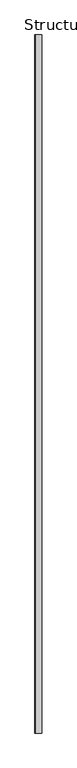
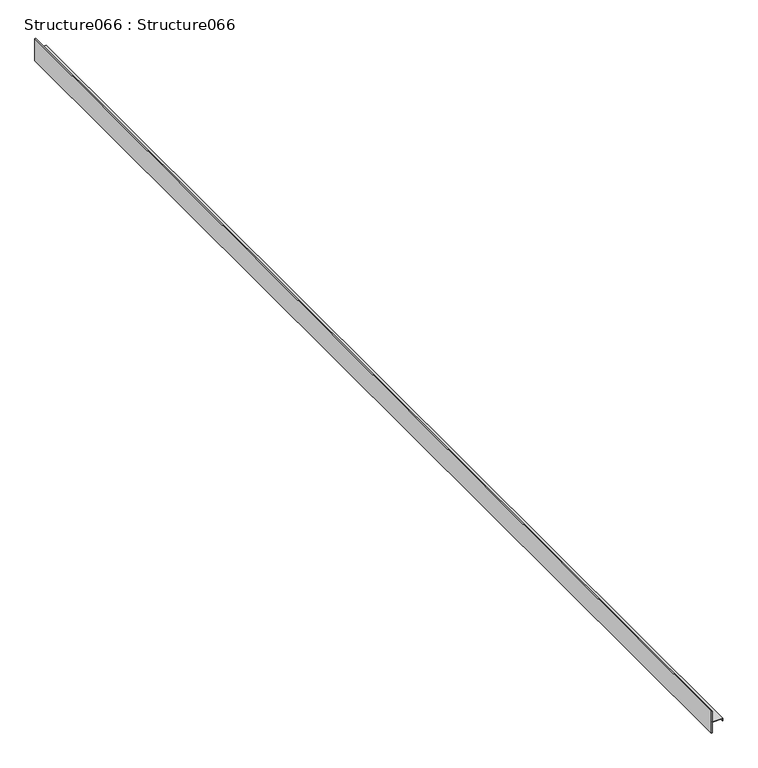
"""IFC4 building model written with IfcOpenShell, lengths in millimetres: proxy geometry, Structure066 : Structure066."""

from ifc_helpers import new_model, si_unit, frame, origin, place, context, project, spatial, polyline, outline, extrude, source, transform, mapped, element, save


def structure066_structure066_e871b1c2(model_context):
    return source(origin(), model_context, "Body", "SweptSolid", [
        extrude(outline(polyline([(40677.3572486, 16522.9406135), (40673.8774486, 16522.9406135), (40673.8774486, 16524.2106135), (40678.6272486, 16524.2106135), (40678.6272486, 16505.9766656), (40697.6772486, 16505.9766656), (40697.6772486, 16504.7066656), (40658.3072486, 16504.7066656), (40658.3072486, 16505.9766656), (40677.3572486, 16505.9766656), (40677.3572486, 16522.9406135)])), frame((0.0, 7982.1435998, 0.0), z_axis=(0.0, 1.0, 0.0), x_axis=(0.0, 0.0, 1.0)), (0.0, 0.0, 1.0), 2000.0),
    ])


if __name__ == "__main__":
    model = new_model("IFC4")
    model_context = context("Model", 3, world=origin())
    ifc_project = project(units=[si_unit("LENGTHUNIT", "METRE", prefix="MILLI")], contexts=[model_context])
    site = spatial("IfcSite", under=ifc_project)
    building = spatial("IfcBuilding", under=site)
    placement = place(None, origin())
    structure066_structure066_shape = structure066_structure066_e871b1c2(model_context)
    element("IfcBuildingElementProxy", 1, Name="Structure066 : Structure066", ObjectType="Structure066 : Structure066", at=placement, inside=building, context=model_context, shape_type="MappedRepresentation", body=[
        mapped(structure066_structure066_shape, transform((0.0, 0.0, 0.0), x_axis=(1.0, 0.0, 0.0), y_axis=(0.0, 1.0, 0.0), z_axis=(0.0, 0.0, 1.0))),
    ])
    save(model, "model.ifc")

# Revit data of these elements
# Type "Structure066 : Structure066"
#   NameOverride = "Structure066"
# Element 1 (IfcBuildingElementProxy, "Structure066 : Structure066")
#   Materials on its faces: "16 GA. COPPER VENTED T REVEAL BEAD"
# Materials
#   "16 GA. COPPER VENTED T REVEAL BEAD": class "Unassigned", colour RGB 255 227 10, transparency 0
